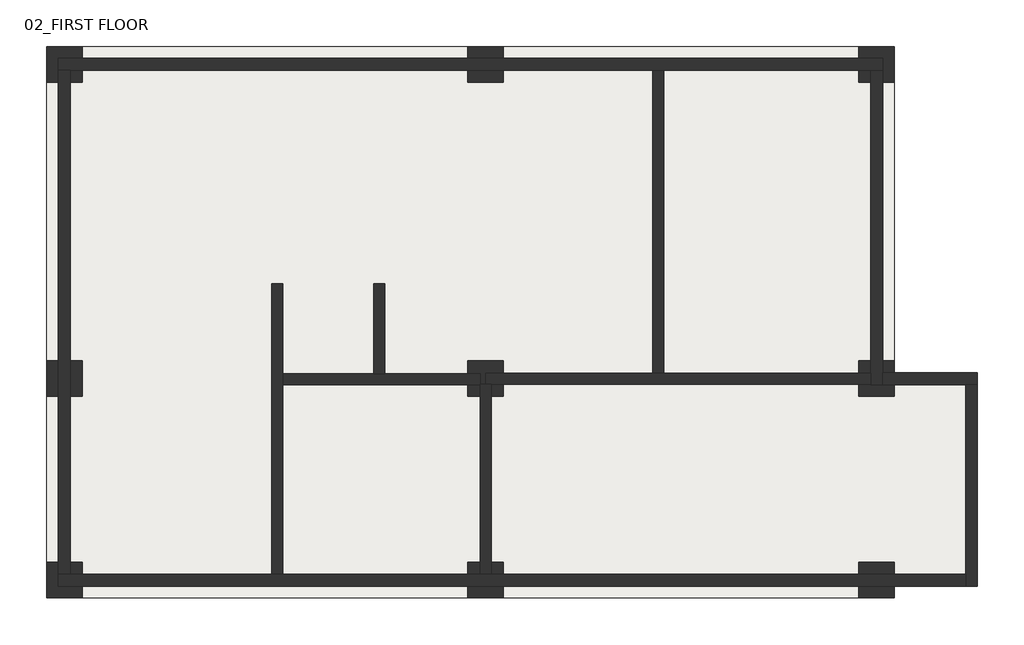
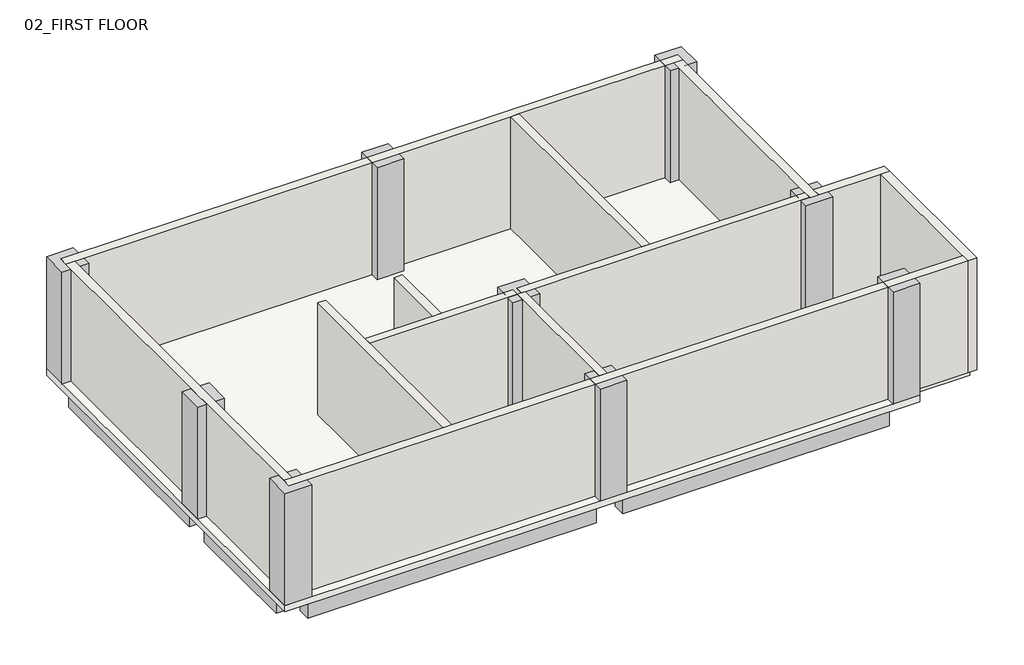
# One storey: 12 beams, 12 walls, 9 columns, 1 slab.
"""IFC4 building model written with IfcOpenShell, lengths in millimetres."""

from ifc_helpers import new_model, si_unit, frame, origin, place, context, project, spatial, polyline, outline, extrude, faceted_brep, element, save

model = new_model("IFC4")

# Units and contexts
model_context = context("Model", 3, world=origin())
ifc_project = project(units=[si_unit("LENGTHUNIT", "METRE", prefix="MILLI")], contexts=[model_context])

# Site, building, storey
site = spatial("IfcSite", under=ifc_project)
building = spatial("IfcBuilding", under=site)
storey = spatial("IfcBuildingStorey", under=building, Name="02_FIRST FLOOR", Elevation=3299.9618634)

# Beams
placement = place(None, origin())
element("IfcBeam", 1, ObjectType="RC Beam_Rectangular : H_SB_AR_S16_B300xH600", at=placement, inside=storey, context=model_context, shape_type="SweptSolid", body=[
    extrude(outline(polyline([(300.0, 1049.5208589), (300.0, 1349.5208589), (6800.0, 1349.5208589), (6800.0, 1049.5208589), (300.0, 1049.5208589)])), frame((0.0, 0.0, 2699.9618634), z_axis=(0.0, 0.0, 1.0), x_axis=(1.0, 0.0, 0.0)), (0.0, 0.0, 1.0), 450.0),
])
element("IfcBeam", 2, ObjectType="RC Beam_Rectangular : H_SB_AR_S16_B300xH600", at=placement, inside=storey, context=model_context, shape_type="SweptSolid", body=[
    extrude(outline(polyline([(7400.0, 1049.5208589), (7400.0, 1349.5208589), (13400.0, 1349.5208589), (13400.0, 1049.5208589), (7400.0, 1049.5208589)])), frame((0.0, 0.0, 2699.9618634), z_axis=(0.0, 0.0, 1.0), x_axis=(1.0, 0.0, 0.0)), (0.0, 0.0, 1.0), 450.0),
])
element("IfcBeam", 3, ObjectType="RC Beam_Rectangular : H_SB_AR_S16_B300xH600", at=placement, inside=storey, context=model_context, shape_type="SweptSolid", body=[
    extrude(outline(polyline([(300.0, 6349.5208589), (300.0, 6649.5208589), (6800.0, 6649.5208589), (6800.0, 6349.5208589), (300.0, 6349.5208589)])), frame((0.0, 0.0, 2699.9618634), z_axis=(0.0, 0.0, 1.0), x_axis=(1.0, 0.0, 0.0)), (0.0, 0.0, 1.0), 450.0),
])
element("IfcBeam", 4, ObjectType="RC Beam_Rectangular : H_SB_AR_S16_B300xH600", at=placement, inside=storey, context=model_context, shape_type="SweptSolid", body=[
    extrude(outline(polyline([(7400.0, 6349.5208589), (7400.0, 6649.5208589), (13400.0, 6649.5208589), (13400.0, 6349.5208589), (7400.0, 6349.5208589)])), frame((0.0, 0.0, 2699.9618634), z_axis=(0.0, 0.0, 1.0), x_axis=(1.0, 0.0, 0.0)), (0.0, 0.0, 1.0), 450.0),
])
element("IfcBeam", 5, ObjectType="RC Beam_Rectangular : H_SB_AR_S16_B300xH600", at=placement, inside=storey, context=model_context, shape_type="SweptSolid", body=[
    extrude(outline(polyline([(300.0, -2350.4791411), (300.0, -2050.4791411), (6800.0, -2050.4791411), (6800.0, -2350.4791411), (300.0, -2350.4791411)])), frame((0.0, 0.0, 2699.9618634), z_axis=(0.0, 0.0, 1.0), x_axis=(1.0, 0.0, 0.0)), (0.0, 0.0, 1.0), 450.0),
])
element("IfcBeam", 6, ObjectType="RC Beam_Rectangular : H_SB_AR_S16_B300xH600", at=placement, inside=storey, context=model_context, shape_type="SweptSolid", body=[
    extrude(outline(polyline([(7400.0, -2350.4791411), (7400.0, -2050.4791411), (13400.0, -2050.4791411), (13400.0, -2350.4791411), (7400.0, -2350.4791411)])), frame((0.0, 0.0, 2699.9618634), z_axis=(0.0, 0.0, 1.0), x_axis=(1.0, 0.0, 0.0)), (0.0, 0.0, 1.0), 450.0),
])
element("IfcBeam", 7, ObjectType="RC Beam_Rectangular : H_SB_AR_S16_B300xH600", at=placement, inside=storey, context=model_context, shape_type="SweptSolid", body=[
    extrude(outline(polyline([(-150.0, 899.5208589), (150.0, 899.5208589), (150.0, -1900.4791411), (-150.0, -1900.4791411), (-150.0, 899.5208589)])), frame((0.0, 0.0, 2699.9618634), z_axis=(0.0, 0.0, 1.0), x_axis=(1.0, 0.0, 0.0)), (0.0, 0.0, 1.0), 450.0),
])
element("IfcBeam", 8, ObjectType="RC Beam_Rectangular : H_SB_AR_S16_B300xH600", at=placement, inside=storey, context=model_context, shape_type="SweptSolid", body=[
    extrude(outline(polyline([(150.0, 1499.5208589), (-150.0, 1499.5208589), (-150.0, 6199.5208589), (150.0, 6199.5208589), (150.0, 1499.5208589)])), frame((0.0, 0.0, 2699.9618634), z_axis=(0.0, 0.0, 1.0), x_axis=(1.0, 0.0, 0.0)), (0.0, 0.0, 1.0), 450.0),
])
element("IfcBeam", 9, ObjectType="RC Beam_Rectangular : H_SB_AR_S16_B300xH600", at=placement, inside=storey, context=model_context, shape_type="SweptSolid", body=[
    extrude(outline(polyline([(6950.0, 899.5208589), (7250.0, 899.5208589), (7250.0, -1900.4791411), (6950.0, -1900.4791411), (6950.0, 899.5208589)])), frame((0.0, 0.0, 2699.9618634), z_axis=(0.0, 0.0, 1.0), x_axis=(1.0, 0.0, 0.0)), (0.0, 0.0, 1.0), 450.0),
])
element("IfcBeam", 10, ObjectType="RC Beam_Rectangular : H_SB_AR_S16_B300xH600", at=placement, inside=storey, context=model_context, shape_type="SweptSolid", body=[
    extrude(outline(polyline([(7250.0, 1499.5208589), (6950.0, 1499.5208589), (6950.0, 6199.5208589), (7250.0, 6199.5208589), (7250.0, 1499.5208589)])), frame((0.0, 0.0, 2699.9618634), z_axis=(0.0, 0.0, 1.0), x_axis=(1.0, 0.0, 0.0)), (0.0, 0.0, 1.0), 450.0),
])
element("IfcBeam", 11, ObjectType="RC Beam_Rectangular : H_SB_AR_S16_B300xH600", at=placement, inside=storey, context=model_context, shape_type="SweptSolid", body=[
    extrude(outline(polyline([(13550.0, 899.5208589), (13850.0, 899.5208589), (13850.0, -1900.4791411), (13550.0, -1900.4791411), (13550.0, 899.5208589)])), frame((0.0, 0.0, 2699.9618634), z_axis=(0.0, 0.0, 1.0), x_axis=(1.0, 0.0, 0.0)), (0.0, 0.0, 1.0), 450.0),
])
element("IfcBeam", 12, ObjectType="RC Beam_Rectangular : H_SB_AR_S16_B300xH600", at=placement, inside=storey, context=model_context, shape_type="SweptSolid", body=[
    extrude(outline(polyline([(13850.0, 1499.5208589), (13550.0, 1499.5208589), (13550.0, 6199.5208589), (13850.0, 6199.5208589), (13850.0, 1499.5208589)])), frame((0.0, 0.0, 2699.9618634), z_axis=(0.0, 0.0, 1.0), x_axis=(1.0, 0.0, 0.0)), (0.0, 0.0, 1.0), 450.0),
])

# Columns
element("IfcColumn", 13, ObjectType="RC_Column_Rectangular : H_SC_AR_S15_W600xL600", at=placement, inside=storey, context=model_context, shape_type="SweptSolid", body=[
    extrude(outline(polyline([(300.0, 1499.5208589), (300.0, 899.5208589), (-300.0, 899.5208589), (-300.0, 1499.5208589), (300.0, 1499.5208589)])), frame((0.0, 0.0, 3299.9618634), z_axis=(0.0, 0.0, 1.0), x_axis=(1.0, 0.0, 0.0)), (0.0, 0.0, 1.0), 2670.0),
])
element("IfcColumn", 14, ObjectType="RC_Column_Rectangular : H_SC_AR_S15_W600xL600", at=placement, inside=storey, context=model_context, shape_type="SweptSolid", body=[
    extrude(outline(polyline([(7400.0, 1499.5208589), (7400.0, 899.5208589), (6800.0, 899.5208589), (6800.0, 1499.5208589), (7400.0, 1499.5208589)])), frame((0.0, 0.0, 3299.9618634), z_axis=(0.0, 0.0, 1.0), x_axis=(1.0, 0.0, 0.0)), (0.0, 0.0, 1.0), 2670.0),
])
element("IfcColumn", 15, ObjectType="RC_Column_Rectangular : H_SC_AR_S15_W600xL600", at=placement, inside=storey, context=model_context, shape_type="SweptSolid", body=[
    extrude(outline(polyline([(14000.0, 1499.5208589), (14000.0, 899.5208589), (13400.0, 899.5208589), (13400.0, 1499.5208589), (14000.0, 1499.5208589)])), frame((0.0, 0.0, 3299.9618634), z_axis=(0.0, 0.0, 1.0), x_axis=(1.0, 0.0, 0.0)), (0.0, 0.0, 1.0), 2670.0),
])
element("IfcColumn", 16, ObjectType="RC_Column_Rectangular : H_SC_AR_S15_W600xL600", at=placement, inside=storey, context=model_context, shape_type="SweptSolid", body=[
    extrude(outline(polyline([(300.0, 6799.5208589), (300.0, 6199.5208589), (-300.0, 6199.5208589), (-300.0, 6799.5208589), (300.0, 6799.5208589)])), frame((0.0, 0.0, 3299.9618634), z_axis=(0.0, 0.0, 1.0), x_axis=(1.0, 0.0, 0.0)), (0.0, 0.0, 1.0), 2670.0),
])
element("IfcColumn", 17, ObjectType="RC_Column_Rectangular : H_SC_AR_S15_W600xL600", at=placement, inside=storey, context=model_context, shape_type="SweptSolid", body=[
    extrude(outline(polyline([(7400.0, 6799.5208589), (7400.0, 6199.5208589), (6800.0, 6199.5208589), (6800.0, 6799.5208589), (7400.0, 6799.5208589)])), frame((0.0, 0.0, 3299.9618634), z_axis=(0.0, 0.0, 1.0), x_axis=(1.0, 0.0, 0.0)), (0.0, 0.0, 1.0), 2670.0),
])
element("IfcColumn", 18, ObjectType="RC_Column_Rectangular : H_SC_AR_S15_W600xL600", at=placement, inside=storey, context=model_context, shape_type="SweptSolid", body=[
    extrude(outline(polyline([(14000.0, 6799.5208589), (14000.0, 6199.5208589), (13400.0, 6199.5208589), (13400.0, 6799.5208589), (14000.0, 6799.5208589)])), frame((0.0, 0.0, 3299.9618634), z_axis=(0.0, 0.0, 1.0), x_axis=(1.0, 0.0, 0.0)), (0.0, 0.0, 1.0), 2670.0),
])
element("IfcColumn", 19, ObjectType="RC_Column_Rectangular : H_SC_AR_S15_W600xL600", at=placement, inside=storey, context=model_context, shape_type="SweptSolid", body=[
    extrude(outline(polyline([(300.0, -1900.4791411), (300.0, -2500.4791411), (-300.0, -2500.4791411), (-300.0, -1900.4791411), (300.0, -1900.4791411)])), frame((0.0, 0.0, 3299.9618634), z_axis=(0.0, 0.0, 1.0), x_axis=(1.0, 0.0, 0.0)), (0.0, 0.0, 1.0), 2670.0),
])
element("IfcColumn", 20, ObjectType="RC_Column_Rectangular : H_SC_AR_S15_W600xL600", at=placement, inside=storey, context=model_context, shape_type="SweptSolid", body=[
    extrude(outline(polyline([(7400.0, -1900.4791411), (7400.0, -2500.4791411), (6800.0, -2500.4791411), (6800.0, -1900.4791411), (7400.0, -1900.4791411)])), frame((0.0, 0.0, 3299.9618634), z_axis=(0.0, 0.0, 1.0), x_axis=(1.0, 0.0, 0.0)), (0.0, 0.0, 1.0), 2670.0),
])
element("IfcColumn", 21, ObjectType="RC_Column_Rectangular : H_SC_AR_S15_W600xL600", at=placement, inside=storey, context=model_context, shape_type="SweptSolid", body=[
    extrude(outline(polyline([(14000.0, -1900.4791411), (14000.0, -2500.4791411), (13400.0, -2500.4791411), (13400.0, -1900.4791411), (14000.0, -1900.4791411)])), frame((0.0, 0.0, 3299.9618634), z_axis=(0.0, 0.0, 1.0), x_axis=(1.0, 0.0, 0.0)), (0.0, 0.0, 1.0), 2670.0),
])

# Slab
element("IfcSlab", 22, ObjectType="H_FL_AR_S17_RC Slab T150", at=placement, inside=storey, context=model_context, shape_type="SweptSolid", body=[
    extrude(outline(polyline([(14000.0, 1199.5208589), (15300.0, 1199.5208589), (15300.0, -2200.4791411), (14000.0, -2200.4791411), (14000.0, -2500.4791411), (-300.0, -2500.4791411), (-300.0, 6799.5208589), (14000.0, 6799.5208589), (14000.0, 1199.5208589)])), frame((0.0, 0.0, 3149.9618634), z_axis=(0.0, 0.0, 1.0), x_axis=(1.0, 0.0, 0.0)), (0.0, 0.0, 1.0), 150.0),
])

# Walls
element("IfcWall", 23, ObjectType="H_WA_AR_B02_Ext Wall_RC T200", at=placement, inside=storey, context=model_context, shape_type="Brep", body=[
    faceted_brep([(-100.0, 6399.5208589, 3299.9618634), (100.0, 6399.5208589, 3299.9618634), (9925.0, 6399.5208589, 3299.9618634), (10109.0, 6399.5208589, 3299.9618634), (13600.0, 6399.5208589, 3299.9618634), (13800.0, 6399.5208589, 3299.9618634), (13800.0, 6399.5208589, 5969.9618634), (13600.0, 6399.5208589, 5969.9618634), (10109.0, 6399.5208589, 5969.9618634), (9925.0, 6399.5208589, 5969.9618634), (100.0, 6399.5208589, 5969.9618634), (-100.0, 6399.5208589, 5969.9618634), (-100.0, 6599.5208589, 3299.9618634), (-100.0, 6599.5208589, 5969.9618634), (13800.0, 6599.5208589, 5969.9618634), (13800.0, 6599.5208589, 3299.9618634)], [[[0, 1, 2, 3, 4, 5, 6, 7, 8, 9, 10, 11]], [[12, 13, 14, 15]], [[5, 4, 3, 2, 1, 0, 12, 15]], [[11, 10, 9, 8, 7, 6, 14, 13]], [[6, 5, 15, 14]], [[0, 11, 13, 12]]]),
])
element("IfcWall", 24, ObjectType="H_WA_AR_B02_Ext Wall_RC T200", at=placement, inside=storey, context=model_context, shape_type="Brep", body=[
    faceted_brep([(13600.0, 6399.5208589, 3299.9618634), (13600.0, 1286.5208589, 3299.9618634), (13600.0, 1102.5208589, 3299.9618634), (13600.0, 1099.5208589, 3299.9618634), (13600.0, 1099.5208589, 5969.9618634), (13600.0, 1102.5208589, 5969.9618634), (13600.0, 1286.5208589, 5969.9618634), (13600.0, 6399.5208589, 5969.9618634), (13800.0, 6399.5208589, 3299.9618634), (13800.0, 6399.5208589, 5969.9618634), (13800.0, 1299.5208589, 5969.9618634), (13800.0, 1099.5208589, 5969.9618634), (13800.0, 1099.5208589, 3299.9618634), (13800.0, 1299.5208589, 3299.9618634)], [[[0, 1, 2, 3, 4, 5, 6, 7]], [[8, 9, 10, 11, 12, 13]], [[3, 2, 1, 0, 8, 13, 12]], [[7, 6, 5, 4, 11, 10, 9]], [[0, 7, 9, 8]], [[4, 3, 12, 11]]]),
])
element("IfcWall", 25, ObjectType="H_WA_AR_B02_Ext Wall_RC T200", at=placement, inside=storey, context=model_context, shape_type="Brep", body=[
    faceted_brep([(13800.0, 1099.5208589, 3299.9618634), (15200.0, 1099.5208589, 3299.9618634), (15400.0, 1099.5208589, 3299.9618634), (15400.0, 1099.5208589, 5969.9618634), (15200.0, 1099.5208589, 5969.9618634), (13800.0, 1099.5208589, 5969.9618634), (13800.0, 1299.5208589, 3299.9618634), (13800.0, 1299.5208589, 5969.9618634), (15400.0, 1299.5208589, 5969.9618634), (15400.0, 1299.5208589, 3299.9618634)], [[[0, 1, 2, 3, 4, 5]], [[6, 7, 8, 9]], [[2, 1, 0, 6, 9]], [[5, 4, 3, 8, 7]], [[0, 5, 7, 6]], [[3, 2, 9, 8]]]),
])
element("IfcWall", 26, ObjectType="H_WA_AR_B02_Ext Wall_RC T200", at=placement, inside=storey, context=model_context, shape_type="Brep", body=[
    faceted_brep([(15200.0, 1099.5208589, 3299.9618634), (15200.0, -2100.4791411, 3299.9618634), (15200.0, -2300.4791411, 3299.9618634), (15200.0, -2300.4791411, 5969.9618634), (15200.0, -2100.4791411, 5969.9618634), (15200.0, 1099.5208589, 5969.9618634), (15400.0, 1099.5208589, 3299.9618634), (15400.0, 1099.5208589, 5969.9618634), (15400.0, -2300.4791411, 5969.9618634), (15400.0, -2300.4791411, 3299.9618634)], [[[0, 1, 2, 3, 4, 5]], [[6, 7, 8, 9]], [[2, 1, 0, 6, 9]], [[5, 4, 3, 8, 7]], [[0, 5, 7, 6]], [[3, 2, 9, 8]]]),
])
element("IfcWall", 27, ObjectType="H_WA_AR_B02_Ext Wall_RC T200", at=placement, inside=storey, context=model_context, shape_type="Brep", body=[
    faceted_brep([(15200.0, -2100.4791411, 3299.9618634), (7197.0, -2100.4791411, 3299.9618634), (7013.0, -2100.4791411, 3299.9618634), (3685.0, -2100.4791411, 3299.9618634), (3501.0, -2100.4791411, 3299.9618634), (100.0, -2100.4791411, 3299.9618634), (-100.0, -2100.4791411, 3299.9618634), (-100.0, -2100.4791411, 5969.9618634), (100.0, -2100.4791411, 5969.9618634), (3501.0, -2100.4791411, 5969.9618634), (3685.0, -2100.4791411, 5969.9618634), (7013.0, -2100.4791411, 5969.9618634), (7197.0, -2100.4791411, 5969.9618634), (15200.0, -2100.4791411, 5969.9618634), (15200.0, -2300.4791411, 3299.9618634), (15200.0, -2300.4791411, 5969.9618634), (-100.0, -2300.4791411, 5969.9618634), (-100.0, -2300.4791411, 3299.9618634)], [[[0, 1, 2, 3, 4, 5, 6, 7, 8, 9, 10, 11, 12, 13]], [[14, 15, 16, 17]], [[6, 5, 4, 3, 2, 1, 0, 14, 17]], [[13, 12, 11, 10, 9, 8, 7, 16, 15]], [[0, 13, 15, 14]], [[7, 6, 17, 16]]]),
])
element("IfcWall", 28, ObjectType="H_WA_AR_B02_Ext Wall_RC T200", at=placement, inside=storey, context=model_context, shape_type="SweptSolid", body=[
    extrude(outline(polyline([(100.0, 6399.5208589), (100.0, -2100.4791411), (-100.0, -2100.4791411), (-100.0, 6399.5208589), (100.0, 6399.5208589)])), frame((0.0, 0.0, 3299.9618634), z_axis=(0.0, 0.0, 1.0), x_axis=(1.0, 0.0, 0.0)), (0.0, 0.0, 1.0), 2670.0),
])
element("IfcWall", 29, ObjectType="H_WA_AR_B02_Int Wall_Block T150", at=placement, inside=storey, context=model_context, shape_type="Brep", body=[
    faceted_brep([(7197.0, -2100.4791411, 3299.9618634), (7197.0, 1102.5208589, 3299.9618634), (7197.0, 1102.5208589, 5969.9618634), (7197.0, -2100.4791411, 5969.9618634), (7013.0, -2100.4791411, 3299.9618634), (7013.0, -2100.4791411, 5969.9618634), (7013.0, 1097.5208589, 5969.9618634), (7013.0, 1102.5208589, 5969.9618634), (7013.0, 1102.5208589, 3299.9618634), (7013.0, 1097.5208589, 3299.9618634), (7105.0, 1102.5208589, 3299.9618634), (7105.0, 1102.5208589, 5969.9618634)], [[[0, 1, 2, 3]], [[4, 5, 6, 7, 8, 9]], [[1, 0, 4, 9, 8, 10]], [[3, 2, 11, 7, 6, 5]], [[0, 3, 5, 4]], [[2, 1, 10, 8, 7, 11]]]),
])
element("IfcWall", 30, ObjectType="H_WA_AR_B02_Int Wall_Block T150", at=placement, inside=storey, context=model_context, shape_type="Brep", body=[
    faceted_brep([(7105.0, 1102.5208589, 3299.9618634), (7197.0, 1102.5208589, 3299.9618634), (13600.0, 1102.5208589, 3299.9618634), (13600.0, 1102.5208589, 5969.9618634), (7197.0, 1102.5208589, 5969.9618634), (7105.0, 1102.5208589, 5969.9618634), (7105.0, 1286.5208589, 3299.9618634), (7105.0, 1286.5208589, 5969.9618634), (9925.0, 1286.5208589, 5969.9618634), (10109.0, 1286.5208589, 5969.9618634), (13600.0, 1286.5208589, 5969.9618634), (13600.0, 1286.5208589, 3299.9618634), (10109.0, 1286.5208589, 3299.9618634), (9925.0, 1286.5208589, 3299.9618634)], [[[0, 1, 2, 3, 4, 5]], [[6, 7, 8, 9, 10, 11, 12, 13]], [[2, 1, 0, 6, 13, 12, 11]], [[5, 4, 3, 10, 9, 8, 7]], [[0, 5, 7, 6]], [[3, 2, 11, 10]]]),
])
element("IfcWall", 31, ObjectType="H_WA_AR_B02_Int Wall_Block T150", at=placement, inside=storey, context=model_context, shape_type="Brep", body=[
    faceted_brep([(3685.0, -2100.4791411, 3299.9618634), (3685.0, 1097.5208589, 3299.9618634), (3685.0, 1281.5208589, 3299.9618634), (3685.0, 2799.5208589, 3299.9618634), (3685.0, 2799.5208589, 5969.9618634), (3685.0, 1281.5208589, 5969.9618634), (3685.0, 1097.5208589, 5969.9618634), (3685.0, -2100.4791411, 5969.9618634), (3501.0, -2100.4791411, 3299.9618634), (3501.0, -2100.4791411, 5969.9618634), (3501.0, 2799.5208589, 5969.9618634), (3501.0, 2799.5208589, 3299.9618634)], [[[0, 1, 2, 3, 4, 5, 6, 7]], [[8, 9, 10, 11]], [[3, 2, 1, 0, 8, 11]], [[4, 3, 11, 10]], [[7, 6, 5, 4, 10, 9]], [[0, 7, 9, 8]]]),
])
element("IfcWall", 32, ObjectType="H_WA_AR_B02_Int Wall_Block T150", at=placement, inside=storey, context=model_context, shape_type="SweptSolid", body=[
    extrude(outline(polyline([(5402.0, 2799.5208589), (5402.0, 1281.5208589), (5218.0, 1281.5208589), (5218.0, 2799.5208589), (5402.0, 2799.5208589)])), frame((0.0, 0.0, 3299.9618634), z_axis=(0.0, 0.0, 1.0), x_axis=(1.0, 0.0, 0.0)), (0.0, 0.0, 1.0), 2670.0),
])
element("IfcWall", 33, ObjectType="H_WA_AR_B02_Int Wall_Block T150", at=placement, inside=storey, context=model_context, shape_type="Brep", body=[
    faceted_brep([(3685.0, 1097.5208589, 3299.9618634), (7013.0, 1097.5208589, 3299.9618634), (7013.0, 1097.5208589, 5969.9618634), (3685.0, 1097.5208589, 5969.9618634), (3685.0, 1281.5208589, 3299.9618634), (3685.0, 1281.5208589, 5969.9618634), (5218.0, 1281.5208589, 5969.9618634), (5402.0, 1281.5208589, 5969.9618634), (7013.0, 1281.5208589, 5969.9618634), (7013.0, 1281.5208589, 3299.9618634), (5402.0, 1281.5208589, 3299.9618634), (5218.0, 1281.5208589, 3299.9618634), (7013.0, 1102.5208589, 3299.9618634), (7013.0, 1102.5208589, 5969.9618634)], [[[0, 1, 2, 3]], [[4, 5, 6, 7, 8, 9, 10, 11]], [[1, 0, 4, 11, 10, 9, 12]], [[3, 2, 13, 8, 7, 6, 5]], [[0, 3, 5, 4]], [[2, 1, 12, 9, 8, 13]]]),
])
element("IfcWall", 34, ObjectType="H_WA_AR_B02_Int Wall_Block T150", at=placement, inside=storey, context=model_context, shape_type="SweptSolid", body=[
    extrude(outline(polyline([(9925.0, 1286.5208589), (9925.0, 6399.5208589), (10109.0, 6399.5208589), (10109.0, 1286.5208589), (9925.0, 1286.5208589)])), frame((0.0, 0.0, 3299.9618634), z_axis=(0.0, 0.0, 1.0), x_axis=(1.0, 0.0, 0.0)), (0.0, 0.0, 1.0), 2670.0),
])

save(model, "model.ifc")

# Revit data of these elements
# Type "RC Beam_Rectangular : H_SB_AR_S16_B300xH600"
#   중앙부 하부근 = ""
#   중앙부 상부근 = ""
#   중앙부 보조근 = ""
#   중앙부 늑근 = ""
#   외단부 하부근 = ""
#   외단부 상부근 = ""
#   외단부 보조근 = ""
#   외단부 늑근 = ""
#   부호 = "TG3"
#   내단부 하부근 = ""
#   내단부 상부근 = ""
#   내단부 보조근 = ""
#   내단부 늑근 = ""
#   ALL 하부근 = "3-D20"
#   ALL 상부근 = "3-D20"
#   ALL 보조근 = ""
#   ALL 늑근 = "2-D10 @120"
#   Width = 300 mm
#   Height = 600 mm
#   Length [instance default] = 1524 mm
#   b = 300 mm
#   h = 600 mm
#   hec_material3 [instance default] = none
#   hec_material2 [instance default] = none
#   hec_material1 [instance default] = none
#   Structural Material [instance default] = none
#   Assembly Code = ""
# Type "RC_Column_Rectangular : H_SC_AR_S15_W600xL600"
#   Width = 600 mm
#   Length = 600 mm
#   hec_material3 [instance default] = none
#   hec_material2 [instance default] = none
#   hec_material1 [instance default] = none
#   Structural Material [instance default] = none
#   Description = (empty or 0)
# Type "H_FL_AR_S17_RC Slab T150"
#   Keynote = ""
#   Type Comments = ""
#   Description = ""
#   Function = 1
#   Layers, outside or top first: 150 mm no material (function 1)
# Type "H_WA_AR_B02_Ext Wall_RC T200"
#   Type Comments = ""
#   Layers, outside or top first: 0 mm no material (function 100); 0 mm no material (function 100); 200 mm no material (function 1); 0 mm no material (function 100); 0 mm no material (function 100); 0 mm no material (function 100)
# Type "H_WA_AR_B02_Int Wall_Block T150"
#   Type Comments = ""
#   Layers, outside or top first: 0 mm no material (function 100); 12 mm no material (function 2); 150 mm no material (function 1); 12 mm no material (function 2); 10 mm no material (function 5)
# Elements 1, 2, 3, 4, 5, 6, 7, 8, 9, 10, 11, 12 (IfcBeam, "RC Beam_Rectangular : H_SB_AR_S16_B300xH600")
#   Comments = ""
#   hec_material3 = none
#   hec_material2 = none
#   hec_material1 = none
#   Structural Material = none
#   Phase Created = New Construction
# Elements 13, 14, 15, 16, 17, 18, 19, 20, 21 (IfcColumn, "RC_Column_Rectangular : H_SC_AR_S15_W600xL600")
#   Comments = ""
#   hec_material3 = none
#   hec_material2 = none
#   hec_material1 = none
#   Structural Material = none
#   Phase Created = New Construction
# Element 22 (IfcSlab, "H_FL_AR_S17_RC Slab T150")
#   Height Offset From Level = 0 mm
#   Phase Created = New Construction
#   Materials on its faces: "Default Floor"
# Elements 23, 24, 25, 26, 27, 28 (IfcWall, "H_WA_AR_B02_Ext Wall_RC T200")
#   Top Offset = 0 mm
#   Base Offset = 0 mm
#   wall height = 2670 mm
#   Phase Created = New Construction
#   Base Constraint = 02_FIRST FLOOR
#   Top Constraint = 03_SECOND FLOOR
#   Materials on its faces: "Default Wall"
# Elements 29, 30, 31, 32, 33, 34 (IfcWall, "H_WA_AR_B02_Int Wall_Block T150")
#   Top Offset = 0 mm
#   Base Offset = 0 mm
#   wall height = 2670 mm
#   Phase Created = New Construction
#   Base Constraint = 02_FIRST FLOOR
#   Top Constraint = 03_SECOND FLOOR
#   Materials on its faces: "Default Wall"
# Materials
#   "Default Floor": class "Miscellaneous", colour RGB 80 80 80, transparency 0
#   "Default Wall": class "Miscellaneous", colour RGB 80 80 80, transparency 0
# Room at (11202.5, -500.479) mm, phase "New Construction", upper level "03_SECOND FLOOR", upper offset 1000 mm, lower offset -1000 mm
#   Comments = ""
#   Number = "130"
#   Name = "STAIRS"
# Room at (5349, -505.479) mm, phase "New Construction", upper level "03_SECOND FLOOR", upper offset 1000 mm, lower offset -1000 mm
#   Comments = ""
#   Number = "131"
#   Name = "TECHNICAL TOWER"
# Room at (11858.5, 3847.021) mm, phase "New Construction", upper level "03_SECOND FLOOR", upper offset 1000 mm, lower offset -1000 mm
#   Comments = ""
#   Number = "132"
#   Name = "LOBBY"
# Room at (5008.5, 2149.521) mm, phase "New Construction", upper level "03_SECOND FLOOR", upper offset 1000 mm, lower offset -1000 mm
#   Comments = ""
#   Number = "133"
#   Name = "CARBONACEOUS FIRE ROOM"
